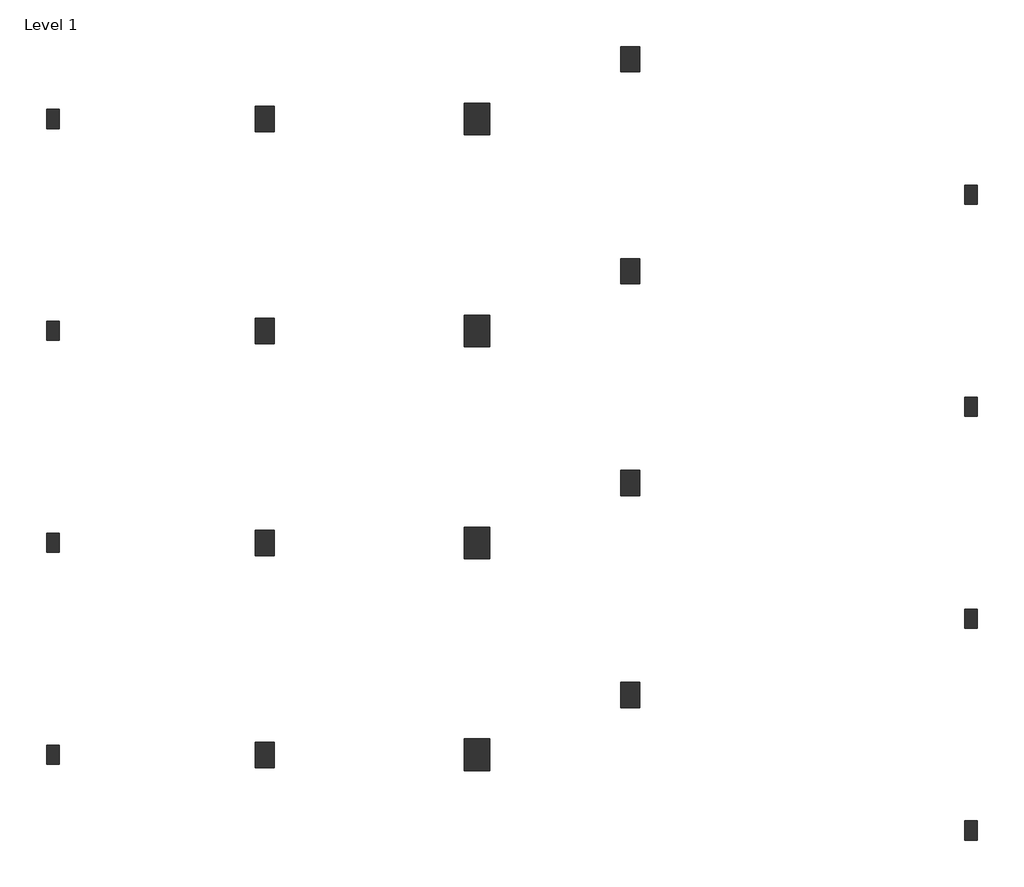
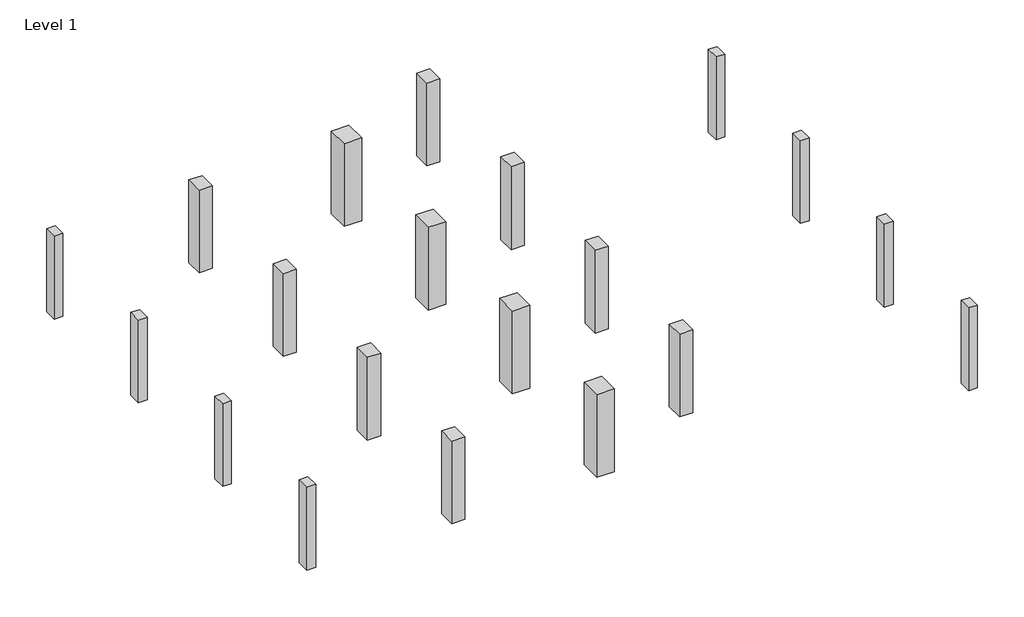
# One storey: 20 columns.
"""IFC4 building model written with IfcOpenShell, lengths in millimetres."""

from ifc_helpers import new_model, si_unit, origin, origin_with_axes, place, context, project, spatial, polyline, outline, extrude, element, save

model = new_model("IFC4")

# Units and contexts
model_context = context("Model", 3, world=origin())
ifc_project = project(units=[si_unit("LENGTHUNIT", "METRE", prefix="MILLI")], contexts=[model_context])

# Site, building, storey
site = spatial("IfcSite", under=ifc_project)
building = spatial("IfcBuilding", under=site)
storey = spatial("IfcBuildingStorey", under=building, Name="Level 1", Elevation=0.0)

# Columns
placement = place(None, origin())
element("IfcColumn", 1, ObjectType="M_Concrete-Rectangular-Column : 300 x 450mm", at=placement, inside=storey, context=model_context, shape_type="SweptSolid", body=[
    extrude(outline(polyline([(-10574.7455739, -9154.7380843), (-10574.7455739, -9604.7380843), (-10874.7455739, -9604.7380843), (-10874.7455739, -9154.7380843), (-10574.7455739, -9154.7380843)])), origin_with_axes(), (0.0, 0.0, 1.0), 3000.0),
])
element("IfcColumn", 2, ObjectType="M_Concrete-Rectangular-Column : 300 x 450mm", at=placement, inside=storey, context=model_context, shape_type="SweptSolid", body=[
    extrude(outline(polyline([(-10574.7455739, -4154.7380843), (-10574.7455739, -4604.7380843), (-10874.7455739, -4604.7380843), (-10874.7455739, -4154.7380843), (-10574.7455739, -4154.7380843)])), origin_with_axes(), (0.0, 0.0, 1.0), 3000.0),
])
element("IfcColumn", 3, ObjectType="M_Concrete-Rectangular-Column : 300 x 450mm", at=placement, inside=storey, context=model_context, shape_type="SweptSolid", body=[
    extrude(outline(polyline([(-10574.7455739, 845.2619157), (-10574.7455739, 395.2619157), (-10874.7455739, 395.2619157), (-10874.7455739, 845.2619157), (-10574.7455739, 845.2619157)])), origin_with_axes(), (0.0, 0.0, 1.0), 3000.0),
])
element("IfcColumn", 4, ObjectType="M_Concrete-Rectangular-Column : 300 x 450mm", at=placement, inside=storey, context=model_context, shape_type="SweptSolid", body=[
    extrude(outline(polyline([(-10574.7455739, 5845.2619157), (-10574.7455739, 5395.2619157), (-10874.7455739, 5395.2619157), (-10874.7455739, 5845.2619157), (-10574.7455739, 5845.2619157)])), origin_with_axes(), (0.0, 0.0, 1.0), 3000.0),
])
element("IfcColumn", 5, ObjectType="M_Concrete-Rectangular-Column : 300 x 450mm", at=placement, inside=storey, context=model_context, shape_type="SweptSolid", body=[
    extrude(outline(polyline([(11084.8320416, -10939.5668406), (11084.8320416, -11389.5668406), (10784.8320416, -11389.5668406), (10784.8320416, -10939.5668406), (11084.8320416, -10939.5668406)])), origin_with_axes(), (0.0, 0.0, 1.0), 3000.0),
])
element("IfcColumn", 6, ObjectType="M_Concrete-Rectangular-Column : 300 x 450mm", at=placement, inside=storey, context=model_context, shape_type="SweptSolid", body=[
    extrude(outline(polyline([(11084.8320416, -5939.5668406), (11084.8320416, -6389.5668406), (10784.8320416, -6389.5668406), (10784.8320416, -5939.5668406), (11084.8320416, -5939.5668406)])), origin_with_axes(), (0.0, 0.0, 1.0), 3000.0),
])
element("IfcColumn", 7, ObjectType="M_Concrete-Rectangular-Column : 300 x 450mm", at=placement, inside=storey, context=model_context, shape_type="SweptSolid", body=[
    extrude(outline(polyline([(11084.8320416, -939.5668406), (11084.8320416, -1389.5668406), (10784.8320416, -1389.5668406), (10784.8320416, -939.5668406), (11084.8320416, -939.5668406)])), origin_with_axes(), (0.0, 0.0, 1.0), 3000.0),
])
element("IfcColumn", 8, ObjectType="M_Concrete-Rectangular-Column : 300 x 450mm", at=placement, inside=storey, context=model_context, shape_type="SweptSolid", body=[
    extrude(outline(polyline([(11084.8320416, 4060.4331594), (11084.8320416, 3610.4331594), (10784.8320416, 3610.4331594), (10784.8320416, 4060.4331594), (11084.8320416, 4060.4331594)])), origin_with_axes(), (0.0, 0.0, 1.0), 3000.0),
])
element("IfcColumn", 9, ObjectType="M_Concrete-Rectangular-Column : 450 x 600mm", at=placement, inside=storey, context=model_context, shape_type="SweptSolid", body=[
    extrude(outline(polyline([(-5499.7455739, -9079.7380843), (-5499.7455739, -9679.7380843), (-5949.7455739, -9679.7380843), (-5949.7455739, -9079.7380843), (-5499.7455739, -9079.7380843)])), origin_with_axes(), (0.0, 0.0, 1.0), 3000.0),
])
element("IfcColumn", 10, ObjectType="M_Concrete-Rectangular-Column : 450 x 600mm", at=placement, inside=storey, context=model_context, shape_type="SweptSolid", body=[
    extrude(outline(polyline([(-5499.7455739, -4079.7380843), (-5499.7455739, -4679.7380843), (-5949.7455739, -4679.7380843), (-5949.7455739, -4079.7380843), (-5499.7455739, -4079.7380843)])), origin_with_axes(), (0.0, 0.0, 1.0), 3000.0),
])
element("IfcColumn", 11, ObjectType="M_Concrete-Rectangular-Column : 450 x 600mm", at=placement, inside=storey, context=model_context, shape_type="SweptSolid", body=[
    extrude(outline(polyline([(-5499.7455739, 920.2619157), (-5499.7455739, 320.2619157), (-5949.7455739, 320.2619157), (-5949.7455739, 920.2619157), (-5499.7455739, 920.2619157)])), origin_with_axes(), (0.0, 0.0, 1.0), 3000.0),
])
element("IfcColumn", 12, ObjectType="M_Concrete-Rectangular-Column : 450 x 600mm", at=placement, inside=storey, context=model_context, shape_type="SweptSolid", body=[
    extrude(outline(polyline([(-5499.7455739, 5920.2619157), (-5499.7455739, 5320.2619157), (-5949.7455739, 5320.2619157), (-5949.7455739, 5920.2619157), (-5499.7455739, 5920.2619157)])), origin_with_axes(), (0.0, 0.0, 1.0), 3000.0),
])
element("IfcColumn", 13, ObjectType="M_Concrete-Rectangular-Column : 450 x 600mm", at=placement, inside=storey, context=model_context, shape_type="SweptSolid", body=[
    extrude(outline(polyline([(3122.4918774, -7670.6627503), (3122.4918774, -8270.6627503), (2672.4918774, -8270.6627503), (2672.4918774, -7670.6627503), (3122.4918774, -7670.6627503)])), origin_with_axes(), (0.0, 0.0, 1.0), 3000.0),
])
element("IfcColumn", 14, ObjectType="M_Concrete-Rectangular-Column : 450 x 600mm", at=placement, inside=storey, context=model_context, shape_type="SweptSolid", body=[
    extrude(outline(polyline([(3122.4918774, -2670.6627503), (3122.4918774, -3270.6627503), (2672.4918774, -3270.6627503), (2672.4918774, -2670.6627503), (3122.4918774, -2670.6627503)])), origin_with_axes(), (0.0, 0.0, 1.0), 3000.0),
])
element("IfcColumn", 15, ObjectType="M_Concrete-Rectangular-Column : 450 x 600mm", at=placement, inside=storey, context=model_context, shape_type="SweptSolid", body=[
    extrude(outline(polyline([(3122.4918774, 2329.3372497), (3122.4918774, 1729.3372497), (2672.4918774, 1729.3372497), (2672.4918774, 2329.3372497), (3122.4918774, 2329.3372497)])), origin_with_axes(), (0.0, 0.0, 1.0), 3000.0),
])
element("IfcColumn", 16, ObjectType="M_Concrete-Rectangular-Column : 450 x 600mm", at=placement, inside=storey, context=model_context, shape_type="SweptSolid", body=[
    extrude(outline(polyline([(3122.4918774, 7329.3372497), (3122.4918774, 6729.3372497), (2672.4918774, 6729.3372497), (2672.4918774, 7329.3372497), (3122.4918774, 7329.3372497)])), origin_with_axes(), (0.0, 0.0, 1.0), 3000.0),
])
element("IfcColumn", 17, ObjectType="M_Concrete-Rectangular-Column : 600 x 750mm", at=placement, inside=storey, context=model_context, shape_type="SweptSolid", body=[
    extrude(outline(polyline([(-424.7455739, -9004.7380843), (-424.7455739, -9754.7380843), (-1024.7455739, -9754.7380843), (-1024.7455739, -9004.7380843), (-424.7455739, -9004.7380843)])), origin_with_axes(), (0.0, 0.0, 1.0), 3000.0),
])
element("IfcColumn", 18, ObjectType="M_Concrete-Rectangular-Column : 600 x 750mm", at=placement, inside=storey, context=model_context, shape_type="SweptSolid", body=[
    extrude(outline(polyline([(-424.7455739, -4004.7380843), (-424.7455739, -4754.7380843), (-1024.7455739, -4754.7380843), (-1024.7455739, -4004.7380843), (-424.7455739, -4004.7380843)])), origin_with_axes(), (0.0, 0.0, 1.0), 3000.0),
])
element("IfcColumn", 19, ObjectType="M_Concrete-Rectangular-Column : 600 x 750mm", at=placement, inside=storey, context=model_context, shape_type="SweptSolid", body=[
    extrude(outline(polyline([(-424.7455739, 995.2619157), (-424.7455739, 245.2619157), (-1024.7455739, 245.2619157), (-1024.7455739, 995.2619157), (-424.7455739, 995.2619157)])), origin_with_axes(), (0.0, 0.0, 1.0), 3000.0),
])
element("IfcColumn", 20, ObjectType="M_Concrete-Rectangular-Column : 600 x 750mm", at=placement, inside=storey, context=model_context, shape_type="SweptSolid", body=[
    extrude(outline(polyline([(-424.7455739, 5995.2619157), (-424.7455739, 5245.2619157), (-1024.7455739, 5245.2619157), (-1024.7455739, 5995.2619157), (-424.7455739, 5995.2619157)])), origin_with_axes(), (0.0, 0.0, 1.0), 3000.0),
])

save(model, "model.ifc")

# Revit data of these elements
# Project information
#   Project Issue Date = "Issue Date"
#   Project Status = "Project Status"
#   Client Name = "Owner"
#   Project Address = "Enter address here"
#   Project Name = "Project Name"
#   Project Number = "Project Number"
# Grids (mm)
#   "1": line (-10724.746, 24350.606) -> (-10724.746, -20955.667)
#   "2": line (-5724.746, 24350.606) -> (-5724.746, -20955.667)
#   "3": line (-724.746, 24350.606) -> (-724.746, -20955.667)
#   "4": line (4275.254, 24350.606) -> (4275.254, -20955.667)
#   "5": line (9275.254, 24350.606) -> (9275.254, -20955.667)
#   "A": line (23306.289, -9379.738) -> (-23847.458, -9379.738)
#   "B": line (23306.289, -4379.738) -> (-23847.458, -4379.738)
#   "C": line (23306.289, 620.262) -> (-23847.458, 620.262)
#   "D": line (23306.289, 5620.262) -> (-23847.458, 5620.262)
# Type "M_Concrete-Rectangular-Column : 300 x 450mm"
#   b = 300 mm
#   h = 450 mm
#   Structural Material [instance default] = Concrete, Cast-in-Place gray
# Type "M_Concrete-Rectangular-Column : 450 x 600mm"
#   b = 450 mm
#   h = 600 mm
#   Structural Material [instance default] = Concrete, Cast-in-Place gray
# Type "M_Concrete-Rectangular-Column : 600 x 750mm"
#   b = 600 mm
#   h = 750 mm
#   Structural Material [instance default] = Concrete, Cast-in-Place gray
# Elements 1, 2, 3, 4, 5, 6, 7, 8 (IfcColumn, "M_Concrete-Rectangular-Column : 300 x 450mm")
#   Structural Material = Concrete, Cast-in-Place gray
#   Phase Created = New Construction
#   Materials on its faces: "Concrete, Cast-in-Place gray"
# Elements 9, 10, 11, 12, 13, 14, 15, 16 (IfcColumn, "M_Concrete-Rectangular-Column : 450 x 600mm")
#   Structural Material = Concrete, Cast-in-Place gray
#   Phase Created = New Construction
#   Materials on its faces: "Concrete, Cast-in-Place gray"
# Elements 17, 18, 19, 20 (IfcColumn, "M_Concrete-Rectangular-Column : 600 x 750mm")
#   Structural Material = Concrete, Cast-in-Place gray
#   Phase Created = New Construction
#   Materials on its faces: "Concrete, Cast-in-Place gray"
# Materials
#   "Concrete, Cast-in-Place gray": class "Concrete", colour RGB 192 192 192, transparency 0, Description = "Cast-in-place concrete", Cost = 0
